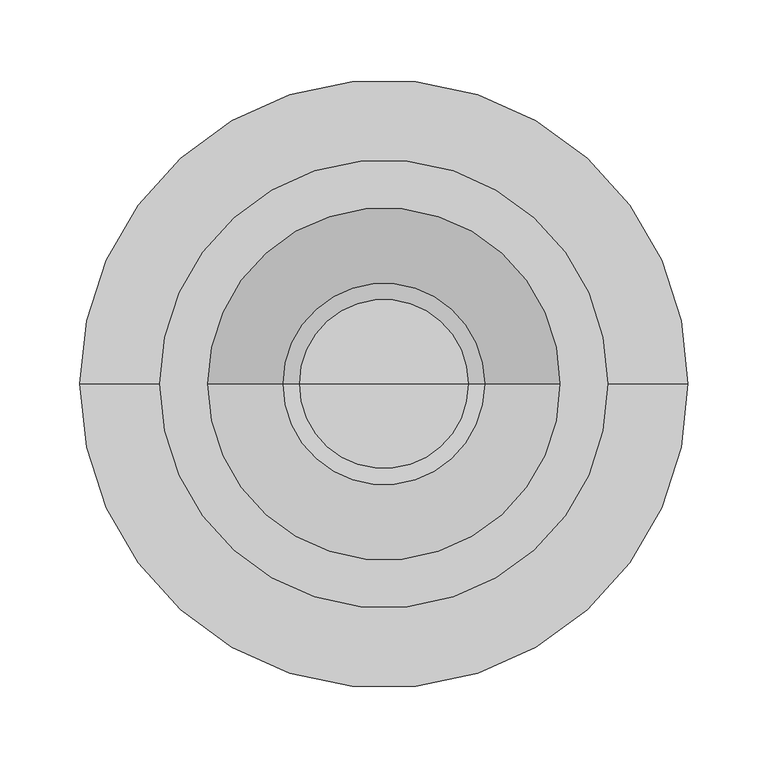
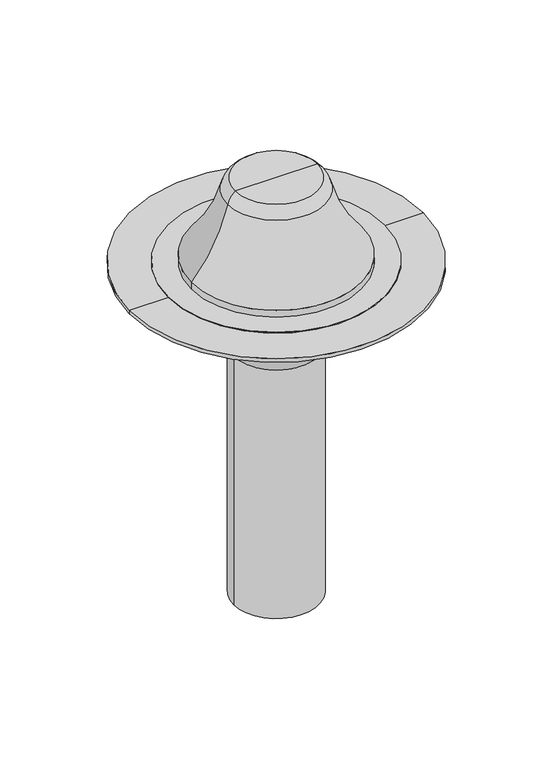
"""IFC4 building model written with IfcOpenShell, lengths in millimetres: proxy geometry, TN_Надставной элемент водоприемной воронки : Надставной элемент с обжимным закручивающемся фланцем и уплотнительным кольцом."""

from ifc_helpers import new_model, si_unit, point, frame, origin, origin_with_axes, origin_2d, place, context, project, spatial, polyline, circle_curve, ellipse_curve, trimmed, segment, composite_curve, outline, extrude, source, transform, mapped, element, save
from ifc_brep_helpers import plane_surface, cylinder_surface, revolved_surface, advanced_brep


def specialty_equipment_ea7c0a3c(model_context):
    return source(origin(), model_context, "Body", "SolidModel", [
        extrude(outline(composite_curve([segment(trimmed(circle_curve(origin_2d(), 140.0), [point((-140.0, 0.0))], [point((140.0, 0.0))], False, "CARTESIAN"), True, "CONTINUOUS"), segment(trimmed(circle_curve(origin_2d(), 140.0), [point((140.0, 0.0))], [point((-140.0, 0.0))], False, "CARTESIAN"), True, "CONTINUOUS")], self_intersect=False), holes=[composite_curve([segment(trimmed(circle_curve(origin_2d(), 110.0556416), [point((-110.0556416, 0.0))], [point((110.0556416, 0.0))], True, "CARTESIAN"), True, "CONTINUOUS"), segment(trimmed(circle_curve(origin_2d(), 110.0556416), [point((110.0556416, 0.0))], [point((-110.0556416, 0.0))], True, "CARTESIAN"), True, "CONTINUOUS")], self_intersect=False)]), origin_with_axes(), (0.0, 0.0, 1.0), 1.0),
        advanced_brep(
        [(110.0556416, 0.0, 0.0), (-110.0556416, 0.0, 0.0), (-110.0556416, 0.0, 10.0), (110.0556416, 0.0, 10.0), (0.0, 0.0, 0.0), (52.7728393, 0.0, 115.0), (-52.7728393, 0.0, 115.0), (0.0, 0.0, 115.0), (62.9807579, 0.0, 100.6532382), (-62.9807579, 0.0, 100.6532382)],
        [
            (0, 1, circle_curve(frame((0.0, 0.0, 0.0), z_axis=(0.0, 0.0, 1.0), x_axis=(-1.0, 0.0, 0.0)), 110.0556416)),
            (1, 2),
            (2, 3, circle_curve(frame((0.0, 0.0, 10.0), z_axis=(0.0, 0.0, -1.0), x_axis=(-1.0, 0.0, 0.0)), 110.0556416)),
            (3, 0),
            (1, 0, circle_curve(frame((0.0, 0.0, 0.0), z_axis=(0.0, 0.0, 1.0), x_axis=(-1.0, 0.0, 0.0)), 110.0556416)),
            (3, 2, circle_curve(frame((0.0, 0.0, 10.0), z_axis=(0.0, 0.0, -1.0), x_axis=(-1.0, 0.0, 0.0)), 110.0556416)),
            (4, 1),
            (0, 4),
            (5, 6, circle_curve(frame((0.0, 0.0, 115.0), z_axis=(0.0, 0.0, 1.0), x_axis=(-1.0, 0.0, 0.0)), 52.7728393)),
            (6, 7),
            (7, 5),
            (6, 5, circle_curve(frame((0.0, 0.0, 115.0), z_axis=(0.0, 0.0, 1.0), x_axis=(-1.0, 0.0, 0.0)), 52.7728393)),
            (8, 9, circle_curve(frame((0.0, 0.0, 100.6532382), z_axis=(0.0, 0.0, 1.0), x_axis=(-1.0, 0.0, 0.0)), 62.9807579)),
            (9, 6, circle_curve(frame((-39.8885443, 0.0, 95.0277285), z_axis=(0.0, 1.0, 0.0), x_axis=(1.0, 0.0, 0.0)), 23.7675553)),
            (5, 8, circle_curve(frame((39.8885443, 0.0, 95.0277285), z_axis=(0.0, 1.0, 0.0), x_axis=(-1.0, 0.0, 0.0)), 23.7675553)),
            (9, 8, circle_curve(frame((0.0, 0.0, 100.6532382), z_axis=(0.0, 0.0, 1.0), x_axis=(-1.0, 0.0, 0.0)), 62.9807579)),
            (2, 9, circle_curve(frame((-271.7387744, 0.0, 151.5089197), z_axis=(0.0, -1.0, 0.0), x_axis=(1.0, 0.0, 0.0)), 214.8632351)),
            (8, 3, circle_curve(frame((271.7387744, 0.0, 151.5089197), z_axis=(0.0, -1.0, 0.0), x_axis=(-1.0, 0.0, 0.0)), 214.8632351)),
        ],
        [
            cylinder_surface(frame((0.0, 0.0, 0.0), z_axis=(0.0, 0.0, -1.0), x_axis=(-1.0, 0.0, 0.0)), 110.0556416),
            plane_surface(frame((0.0, 0.0, 0.0), z_axis=(0.0, 0.0, -1.0), x_axis=(-1.0, 0.0, 0.0))),
            plane_surface(frame((0.0, 0.0, 115.0), z_axis=(0.0, 0.0, 1.0), x_axis=(-1.0, 0.0, 0.0))),
            revolved_surface(trimmed(ellipse_curve(frame((-39.8885443, 0.0, 95.0277285), z_axis=(0.0, -1.0, 0.0), x_axis=(1.0, 0.0, 0.0)), 23.7675553, 23.7675553), [point((-52.7728393, 0.0, 115.0))], [point((-62.9807579, 0.0, 100.6532382))], True, "CARTESIAN"), (0.0, 0.0, 0.0), (0.0, 0.0, -1.0)),
            revolved_surface(trimmed(ellipse_curve(frame((-271.7387744, 0.0, 151.5089197), z_axis=(0.0, 1.0, 0.0), x_axis=(1.0, 0.0, 0.0)), 214.8632351, 214.8632351), [point((-62.9807579, 0.0, 100.6532382))], [point((-110.0556416, 0.0, 10.0))], True, "CARTESIAN"), (0.0, 0.0, 0.0), (0.0, 0.0, -1.0)),
        ],
        [
            (0, [[1, 2, 3, 4]]),
            (0, [[5, -4, 6, -2]]),
            (1, [[7, -1, 8]]),
            (1, [[-8, -5, -7]]),
            (2, [[9, 10, 11]]),
            (2, [[12, -11, -10]]),
            (3, [[13, 14, -9, 15]]),
            (3, [[16, -15, -12, -14]]),
            (4, [[-3, 17, -13, 18]]),
            (4, [[-6, -18, -16, -17]]),
        ],
    ),
        advanced_brep(
        [(0.0, 0.0, -450.0), (-55.0, 0.0, -450.0), (55.0, 0.0, -450.0), (190.0, 0.0, 0.0), (-190.0, 0.0, 0.0), (-83.890873, 0.0, 0.0), (83.890873, 0.0, 0.0), (190.0, 0.0, -5.0), (-190.0, 0.0, -5.0), (93.890873, 0.0, -5.0), (-93.890873, 0.0, -5.0), (55.0, 0.0, -110.0), (-55.0, 0.0, -110.0), (-93.890873, 0.0, -71.109127), (93.890873, 0.0, -71.109127), (55.5025253, 0.0, -95.3553391), (-55.5025253, 0.0, -95.3553391), (0.0, 0.0, -95.3553391), (83.890873, 0.0, -66.9669914), (-83.890873, 0.0, -66.9669914)],
        [
            (0, 1),
            (1, 2, circle_curve(frame((0.0, 0.0, -450.0), z_axis=(0.0, 0.0, -1.0), x_axis=(-1.0, 0.0, 0.0)), 55.0)),
            (2, 0),
            (2, 1, circle_curve(frame((0.0, 0.0, -450.0), z_axis=(0.0, 0.0, -1.0), x_axis=(-1.0, 0.0, 0.0)), 55.0)),
            (3, 4, circle_curve(frame((0.0, 0.0, 0.0), z_axis=(0.0, 0.0, 1.0), x_axis=(-1.0, 0.0, 0.0)), 190.0)),
            (4, 5),
            (5, 6, circle_curve(frame((0.0, 0.0, 0.0), z_axis=(0.0, 0.0, -1.0), x_axis=(-1.0, 0.0, 0.0)), 83.890873)),
            (6, 3),
            (4, 3, circle_curve(frame((0.0, 0.0, 0.0), z_axis=(0.0, 0.0, 1.0), x_axis=(-1.0, 0.0, 0.0)), 190.0)),
            (6, 5, circle_curve(frame((0.0, 0.0, 0.0), z_axis=(0.0, 0.0, -1.0), x_axis=(-1.0, 0.0, 0.0)), 83.890873)),
            (7, 8, circle_curve(frame((0.0, 0.0, -5.0), z_axis=(0.0, 0.0, 1.0), x_axis=(-1.0, 0.0, 0.0)), 190.0)),
            (8, 4),
            (3, 7),
            (8, 7, circle_curve(frame((0.0, 0.0, -5.0), z_axis=(0.0, 0.0, 1.0), x_axis=(-1.0, 0.0, 0.0)), 190.0)),
            (9, 10, circle_curve(frame((0.0, 0.0, -5.0), z_axis=(0.0, 0.0, 1.0), x_axis=(-1.0, 0.0, 0.0)), 93.890873)),
            (10, 8),
            (7, 9),
            (10, 9, circle_curve(frame((0.0, 0.0, -5.0), z_axis=(0.0, 0.0, 1.0), x_axis=(-1.0, 0.0, 0.0)), 93.890873)),
            (11, 12, circle_curve(frame((0.0, 0.0, -110.0), z_axis=(0.0, 0.0, 1.0), x_axis=(-1.0, 0.0, 0.0)), 55.0)),
            (12, 13),
            (13, 14, circle_curve(frame((0.0, 0.0, -71.109127), z_axis=(0.0, 0.0, -1.0), x_axis=(-1.0, 0.0, 0.0)), 93.890873)),
            (14, 11),
            (12, 11, circle_curve(frame((0.0, 0.0, -110.0), z_axis=(0.0, 0.0, 1.0), x_axis=(-1.0, 0.0, 0.0)), 55.0)),
            (14, 13, circle_curve(frame((0.0, 0.0, -71.109127), z_axis=(0.0, 0.0, -1.0), x_axis=(-1.0, 0.0, 0.0)), 93.890873)),
            (1, 12),
            (11, 2),
            (13, 10),
            (9, 14),
            (15, 16, circle_curve(frame((0.0, 0.0, -95.3553391), z_axis=(0.0, 0.0, 1.0), x_axis=(-1.0, 0.0, 0.0)), 55.5025253)),
            (16, 17),
            (17, 15),
            (16, 15, circle_curve(frame((0.0, 0.0, -95.3553391), z_axis=(0.0, 0.0, 1.0), x_axis=(-1.0, 0.0, 0.0)), 55.5025253)),
            (18, 19, circle_curve(frame((0.0, 0.0, -66.9669914), z_axis=(0.0, 0.0, 1.0), x_axis=(-1.0, 0.0, 0.0)), 83.890873)),
            (19, 16),
            (15, 18),
            (19, 18, circle_curve(frame((0.0, 0.0, -66.9669914), z_axis=(0.0, 0.0, 1.0), x_axis=(-1.0, 0.0, 0.0)), 83.890873)),
            (5, 19),
            (18, 6),
        ],
        [
            plane_surface(frame((0.0, 0.0, -450.0), z_axis=(0.0, 0.0, -1.0), x_axis=(-1.0, 0.0, 0.0))),
            plane_surface(frame((0.0, 0.0, 0.0), z_axis=(0.0, 0.0, 1.0), x_axis=(-1.0, 0.0, 0.0))),
            cylinder_surface(frame((0.0, 0.0, 0.0), z_axis=(0.0, 0.0, -1.0), x_axis=(-1.0, 0.0, 0.0)), 190.0),
            plane_surface(frame((0.0, 0.0, -5.0), z_axis=(0.0, 0.0, -1.0), x_axis=(-1.0, 0.0, 0.0))),
            revolved_surface(polyline([(-93.890873, 0.0, -71.109127), (-55.0, 0.0, -110.0)]), (0.0, 0.0, 0.0), (0.0, 0.0, -1.0)),
            cylinder_surface(frame((0.0, 0.0, 0.0), z_axis=(0.0, 0.0, -1.0), x_axis=(-1.0, 0.0, 0.0)), 55.0),
            cylinder_surface(frame((0.0, 0.0, 0.0), z_axis=(0.0, 0.0, -1.0), x_axis=(-1.0, 0.0, 0.0)), 93.890873),
            plane_surface(frame((0.0, 0.0, -95.3553391), z_axis=(0.0, 0.0, 1.0), x_axis=(-1.0, 0.0, 0.0))),
            revolved_surface(polyline([(-55.5025253, 0.0, -95.3553391), (-83.890873, 0.0, -66.9669914)]), (0.0, 0.0, 0.0), (0.0, 0.0, -1.0)),
            revolved_surface(polyline([(-83.890873, 0.0, -66.9669914), (-83.890873, 0.0, 0.0)]), (0.0, 0.0, 0.0), (0.0, 0.0, -1.0)),
        ],
        [
            (0, [[1, 2, 3]]),
            (0, [[-3, 4, -1]]),
            (1, [[5, 6, 7, 8]]),
            (1, [[9, -8, 10, -6]]),
            (2, [[11, 12, -5, 13]]),
            (2, [[14, -13, -9, -12]]),
            (3, [[15, 16, -11, 17]]),
            (3, [[18, -17, -14, -16]]),
            (4, [[19, 20, 21, 22]]),
            (4, [[23, -22, 24, -20]]),
            (5, [[-2, 25, -19, 26]]),
            (5, [[-4, -26, -23, -25]]),
            (6, [[-21, 27, -15, 28]]),
            (6, [[-24, -28, -18, -27]]),
            (7, [[29, 30, 31]]),
            (7, [[32, -31, -30]]),
            (8, [[33, 34, -29, 35]]),
            (8, [[36, -35, -32, -34]]),
            (9, [[-7, 37, -33, 38]]),
            (9, [[-10, -38, -36, -37]]),
        ],
    ),
    ])


if __name__ == "__main__":
    model = new_model("IFC4")
    model_context = context("Model", 3, world=origin())
    ifc_project = project(units=[si_unit("LENGTHUNIT", "METRE", prefix="MILLI")], contexts=[model_context])
    site = spatial("IfcSite", under=ifc_project)
    building = spatial("IfcBuilding", under=site)
    placement = place(None, origin())
    specialty_equipment_shape = specialty_equipment_ea7c0a3c(model_context)
    element("IfcBuildingElementProxy", 1, Name="TN_Надставной элемент водоприемной воронки : Надставной элемент с обжимным закручивающемся фланцем и уплотнительным кольцом", ObjectType="TN_Надставной элемент водоприемной воронки : Надставной элемент с обжимным закручивающемся фланцем и уплотнительным кольцом", at=placement, inside=building, context=model_context, shape_type="MappedRepresentation", body=[
        mapped(specialty_equipment_shape, transform((0.0, 0.0, 0.0), x_axis=(1.0, 0.0, 0.0), y_axis=(0.0, 1.0, 0.0), z_axis=(0.0, 0.0, 1.0))),
    ])
    save(model, "model.ifc")

# Revit data of these elements
# Type "TN_Надставной элемент водоприемной воронки : Надставной элемент с обжимным закручивающемся фланцем и уплотнительным кольцом"
#   ADSK_Группирование = "Комплектующие и воронки"
#   Description = "Надставной элемент с обжимным металлическим фланцем и уплотнительным кольцом применяется для создания двух уровневых кровельных воронок. Манжета предотвращает проникновение ливневых стоков в слой теплоизоляции по месту соединения надставного элемента с воронкой. Может быть также использован как самостоятельное изделие подобно воронке с обжимным металлическим фланцем. Также надставной элемент комплектуется уплотнительным кольцом, комплектом гаек и барашков."
#   Manufacturer = "ТехноНИКОЛЬ"
#   URL = "https://shop.tn.ru/nadstavnoj-jelement-s-obzhimnym-zakruchivajuschemsja-flancem-i-uplotnitelnym-kolcom"
#   ADSK_Примечание = ""
#   ADSK_Обозначение = "ТехноНИКОЛЬ"
#   ADSK_Наименование = "Надставной элемент с обжимным закручивающемся  фланцем и уплотнительным кольцом"
#   ADSK_Марка = ""
#   ADSK_Код изделия = "661129"
#   ADSK_Завод-изготовитель = "ТехноНИКОЛЬ"
#   ADSK_Единица измерения = "шт."
#   ADSK_Группирование = "Комплектующие и воронки"
#   ADSK_URL страницы изделия = "https://shop.tn.ru/nadstavnoj-jelement-s-obzhimnym-zakruchivajuschemsja-flancem-i-uplotnitelnym-kolcom"
#   ADSK_URL документации изделия = "https://shop.tn.ru/media/other_documents/_661129_661126_661128_661127_661133_1.pdf"
#   Тип надставного элемента = 1
#   Радиус = 55 mm
#   Длина расчетная [instance default] = 450 mm
#   Длина отвода [instance default] = 450 mm
#   Высота трапа расчетная [instance default] = 51 mm
#   Высота трапа [instance default] = 51 mm
#   ADSK_Количество = 1
#   Видимость_Листоуловитель [instance default] = yes
#   Видимость трапа [instance default] = no
#   Видимость листоуловителя [instance default] = yes
#   Материал_Фланец = TN_Фланец_Красный
#   Материал_Корпус = TN_ПВХ_Черный
#   Default Elevation = 0
# Element 1 (IfcBuildingElementProxy, "TN_Надставной элемент водоприемной воронки : Надставной элемент с обжимным закручивающемся фланцем и уплотнительным кольцом")
#   Высота трапа расчетная = 50 mm
#   Высота трапа = 0 mm
#   Materials on its faces: "TN_ПВХ_Черный", "TN_Фланец_Красный"
# Materials
#   "TN_Фланец_Красный": class "Типовые", colour RGB 70 0 0, transparency 0, Cost = 0
#   "TN_ПВХ_Черный": class "Типовые", colour RGB 48 48 48, transparency 0, Cost = 0
